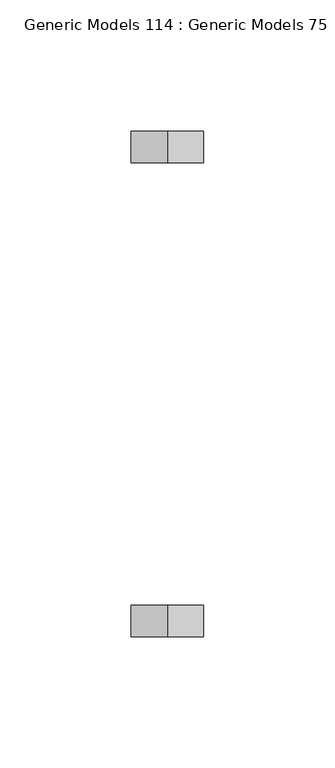
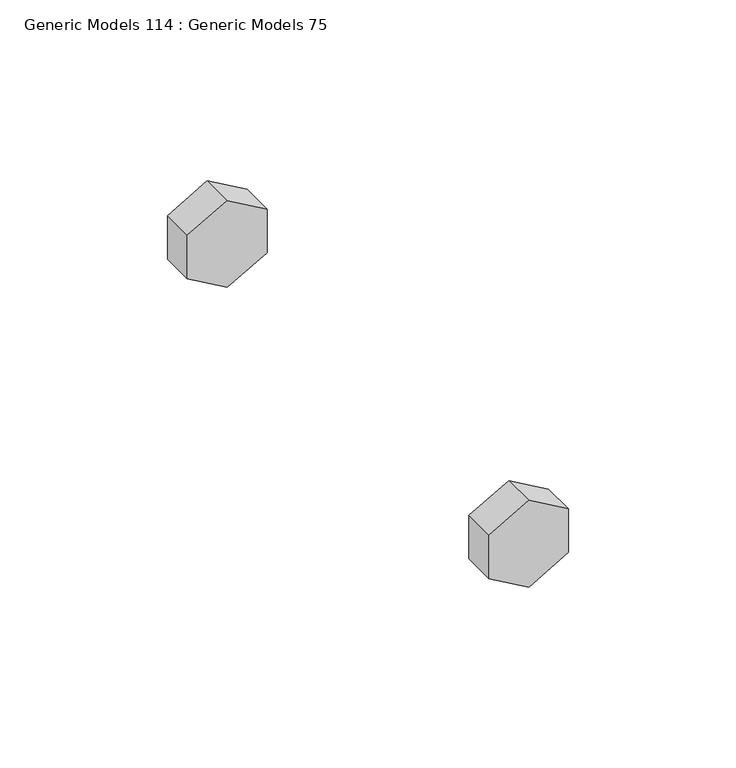
"""IFC4 building model written with IfcOpenShell, lengths in millimetres: proxy geometry, Generic Models 114 : Generic Models 75."""

from ifc_helpers import new_model, si_unit, frame, origin, place, context, project, spatial, polyline, outline, extrude, source, transform, mapped, element, save


def generic_models_114_generic_models_75_769741ad(model_context):
    return source(origin(), model_context, "Body", "SweptSolid", [
        extrude(outline(polyline([(269222.3462802, 31975.9942029), (269206.5097067, 31975.9942029), (269198.59142, 31989.7090778), (269206.5097067, 32003.4239528), (269222.3462802, 32003.4239528), (269230.264567, 31989.7090778), (269222.3462802, 31975.9942029)])), frame((0.0, 35373.9582942, 0.0), z_axis=(0.0, 1.0, 0.0), x_axis=(0.0, 0.0, 1.0)), (0.0, 0.0, 1.0), 11.90625),
        extrude(outline(polyline([(269222.3462802, 31975.9942029), (269206.5097067, 31975.9942029), (269198.59142, 31989.7090778), (269206.5097067, 32003.4239528), (269222.3462802, 32003.4239528), (269230.264567, 31989.7090778), (269222.3462802, 31975.9942029)])), frame((0.0, 35193.7770442, 0.0), z_axis=(0.0, 1.0, 0.0), x_axis=(0.0, 0.0, 1.0)), (0.0, 0.0, 1.0), 11.90625),
    ])


if __name__ == "__main__":
    model = new_model("IFC4")
    model_context = context("Model", 3, world=origin())
    ifc_project = project(units=[si_unit("LENGTHUNIT", "METRE", prefix="MILLI")], contexts=[model_context])
    site = spatial("IfcSite", under=ifc_project)
    building = spatial("IfcBuilding", under=site)
    placement = place(None, origin())
    generic_models_114_generic_models_75_shape = generic_models_114_generic_models_75_769741ad(model_context)
    element("IfcBuildingElementProxy", 1, Name="Generic Models 114 : Generic Models 75", ObjectType="Generic Models 114 : Generic Models 75", at=placement, inside=building, context=model_context, shape_type="MappedRepresentation", body=[
        mapped(generic_models_114_generic_models_75_shape, transform((0.0, 0.0, 0.0), x_axis=(1.0, 0.0, 0.0), y_axis=(0.0, 1.0, 0.0), z_axis=(0.0, 0.0, 1.0))),
    ])
    save(model, "model.ifc")

# Revit data of these elements
# Element 1 (IfcBuildingElementProxy, "Generic Models 114 : Generic Models 75")
#   Materials on its faces: "3/4\" GALV. THRU BOLTS"
# Materials
#   "3/4\" GALV. THRU BOLTS": class "Generic", colour RGB 105 69 171, transparency 0, Cost = 0
